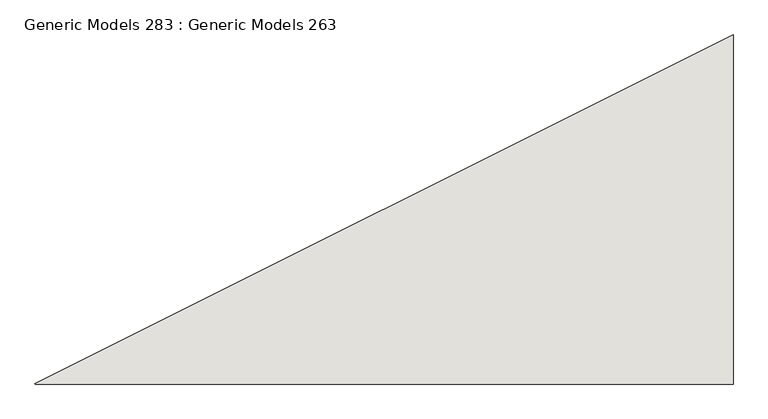
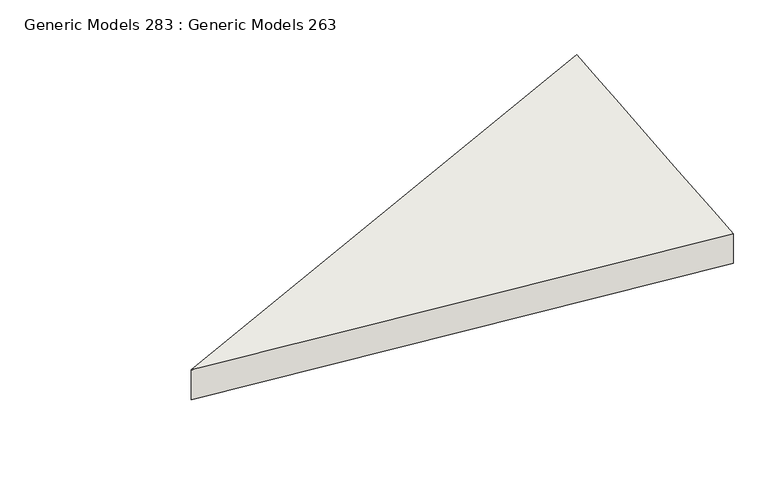
"""IFC4 building model written with IfcOpenShell, lengths in millimetres: wall geometry, Generic Models 283 : Generic Models 263."""

from ifc_helpers import new_model, si_unit, frame, origin, place, context, project, spatial, source, transform, mapped, element, save
from ifc_brep_helpers import plane_surface, spline_surface, advanced_brep


def generic_models_283_generic_models_263_7587e6aa(model_context):
    return source(origin(), model_context, "Body", "AdvancedBrep", [
        advanced_brep(
        [(269252.9797726, 2106.5727422, 2.0699085), (269252.9797726, 582.5727422, -137.0198762), (269252.9797726, 582.5727422, -314.8198762), (269252.9797726, 2106.5727422, -314.8198762), (266204.9797726, 583.7192284, 120.3150752), (266204.9797726, 583.7192284, -58.1173502), (266204.9797726, 582.5727422, -58.1173502), (266204.9797726, 582.5727422, 120.3150752)],
        [
            (0, 1),
            (1, 2),
            (2, 3),
            (3, 0),
            (4, 5),
            (5, 6),
            (6, 7),
            (7, 4),
            (4, 0),
            (3, 5),
            (2, 6),
            (1, 7),
        ],
        [
            plane_surface(frame((269252.9797726, 1344.5727422, -191.14743), z_axis=(1.0, 0.0, 0.0), x_axis=(0.0, -0.9958610732446469, -0.09088851850492481))),
            plane_surface(frame((266204.9797726, 583.1459853, 31.0988625), z_axis=(-1.0, 0.0, 0.0), x_axis=(0.0, -0.9958610732446469, -0.09088851850492481))),
            plane_surface(frame((266204.9797726, 583.7192284, 31.0988625), z_axis=(-0.44694438819938426, 0.894561744016073, 0.0), x_axis=(0.0, 0.0, 1.0))),
            plane_surface(frame((266204.9797726, 583.1459853, -58.1173502), z_axis=(-0.08392288197547106, 0.0, -0.9964722524390387), x_axis=(0.0, 1.0, 0.0))),
            plane_surface(frame((266204.9797726, 582.5727422, 31.0988625), z_axis=(0.0, -1.0, 0.0), x_axis=(0.0, 0.0, -1.0))),
            spline_surface(1, 1, [[(266204.9797726, 583.7192284, 120.3150752), (269252.9797726, 2106.5727422, 2.0699085)], [(266204.9797726, 582.5727422, 120.3150752), (269252.9797726, 582.5727422, -137.0198762)]], [2, 2], [2, 2], [0.0, 1.0], [0.0, 1.0]),
        ],
        [
            (0, [[1, 2, 3, 4]]),
            (1, [[5, 6, 7, 8]]),
            (2, [[-5, 9, -4, 10]]),
            (3, [[-6, -10, -3, 11]]),
            (4, [[-7, -11, -2, 12]]),
            (5, [[-8, -12, -1, -9]]),
        ],
    ),
    ])


if __name__ == "__main__":
    model = new_model("IFC4")
    model_context = context("Model", 3, world=origin())
    ifc_project = project(units=[si_unit("LENGTHUNIT", "METRE", prefix="MILLI")], contexts=[model_context])
    site = spatial("IfcSite", under=ifc_project)
    building = spatial("IfcBuilding", under=site)
    placement = place(None, origin())
    generic_models_283_generic_models_263_shape = generic_models_283_generic_models_263_7587e6aa(model_context)
    element("IfcWall", 1, ObjectType="Generic Models 283 : Generic Models 263", at=placement, inside=building, context=model_context, shape_type="MappedRepresentation", body=[
        mapped(generic_models_283_generic_models_263_shape, transform((0.0, 0.0, 0.0), x_axis=(1.0, 0.0, 0.0), y_axis=(0.0, 1.0, 0.0), z_axis=(0.0, 0.0, 1.0))),
    ])
    save(model, "model.ifc")

# Revit data of these elements
# Element 1 (IfcWall, "Generic Models 283 : Generic Models 263")
#   Materials on its faces: "SLOPED - 7\" CONC."
# Materials
#   "SLOPED - 7\" CONC.": class "Concrete", colour RGB 191 191 191, transparency 0, Description = "Cast-in-place concrete", Cost = 0
